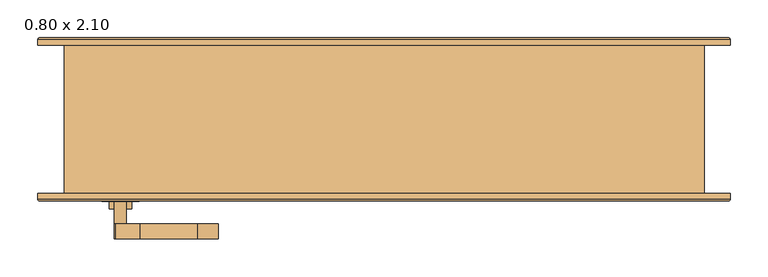
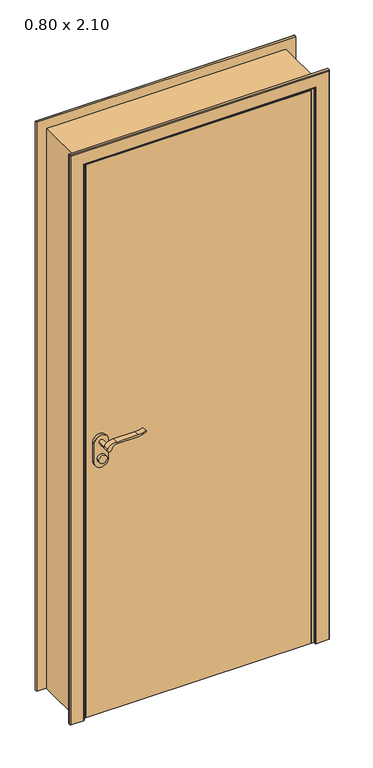
"""IFC4 building model written with IfcOpenShell, lengths in millimetres: door geometry, .CC_ND 300_PORTA SIMPLES DE ABRIR_COM EXTENSÃO : 0.80 x 2.10."""

import ifcopenshell
import ifcopenshell.guid

model = None  # the IFC model being written
_history = None  # IfcOwnerHistory: only IFC2X3 demands one
_inside = {}  # id of a spatial element -> (the spatial element, [elements in it])
_under = {}  # id of a project, library or spatial element -> (it, [spatial elements below it])
_declared = {}  # id of a project -> (the project, [libraries it declares])
_typed = {}  # id of a type object -> (the type object, [elements of that type])
_made_of = {}  # id of a material, layer set ... -> (it, [elements and type objects made of it])


def new_model(schema):
    """Start an empty IFC model of exactly this schema.

    Asked for "IFC4X3", IfcOpenShell would pick the latest addendum, in which some entities
    have other attributes; the version numbers below select the first issue.
    IFC2X3 requires an IfcOwnerHistory on every rooted entity: one is made here for all.
    """
    global model, _history
    if schema == "IFC4X3":
        model = ifcopenshell.file(schema_version=(4, 3, 0, 0))
    else:
        model = ifcopenshell.file(schema=schema)
    _inside.clear()
    _under.clear()
    _declared.clear()
    _typed.clear()
    _made_of.clear()
    _history = None
    if model.schema == "IFC2X3":
        org = make("IfcOrganization", Name="unknown")
        user = make(
            "IfcPersonAndOrganization",
            ThePerson=make("IfcPerson", FamilyName="unknown"),
            TheOrganization=org,
        )
        app = make(
            "IfcApplication",
            ApplicationDeveloper=org,
            Version="unknown",
            ApplicationFullName="unknown",
            ApplicationIdentifier="unknown",
        )
        _history = make(
            "IfcOwnerHistory",
            OwningUser=user,
            OwningApplication=app,
            ChangeAction="ADDED",
            CreationDate=0,
        )
    return model


def make(cls, **values):
    """One entity of the class cls with the attributes given. An attribute that is None is left unset."""
    return model.create_entity(
        cls, **{name: value for name, value in values.items() if value is not None}
    )


def rooted(cls, **values):
    """An entity with a GlobalId (a new one), such as an element, a storey or a relation."""
    return make(cls, GlobalId=ifcopenshell.guid.new(), OwnerHistory=_history, **values)


def si_unit(unit_type, name, prefix=None):
    """IfcSIUnit, for example si_unit("LENGTHUNIT", "METRE", prefix="MILLI")."""
    return make("IfcSIUnit", UnitType=unit_type, Prefix=prefix, Name=name)


def assignment(units):
    """IfcUnitAssignment: the units of a project."""
    return None if units is None else make("IfcUnitAssignment", Units=units)


def point(xyz):
    """IfcCartesianPoint."""
    return None if xyz is None else make("IfcCartesianPoint", Coordinates=xyz)


def direction(xyz):
    """IfcDirection."""
    return None if xyz is None else make("IfcDirection", DirectionRatios=xyz)


def frame(location, z_axis=None, x_axis=None):
    """IfcAxis2Placement3D, a coordinate frame: its origin and axes. An axis left out is left unset."""
    return make(
        "IfcAxis2Placement3D",
        Location=point(location),
        Axis=direction(z_axis),
        RefDirection=direction(x_axis),
    )


def frame_2d(location, x_axis=None):
    """IfcAxis2Placement2D, a coordinate frame in the plane: its origin and x axis."""
    return make(
        "IfcAxis2Placement2D", Location=point(location), RefDirection=direction(x_axis)
    )


def origin():
    """The frame at (0, 0, 0) with its axes left unset."""
    return frame((0.0, 0.0, 0.0))


def origin_with_axes():
    """The frame at (0, 0, 0) with the z axis (0, 0, 1) and the x axis (1, 0, 0) written out."""
    return frame((0.0, 0.0, 0.0), z_axis=(0.0, 0.0, 1.0), x_axis=(1.0, 0.0, 0.0))


def place(relative_to, where):
    """IfcLocalPlacement: puts the frame where relative to a parent placement (None: the world)."""
    return make(
        "IfcLocalPlacement", PlacementRelTo=relative_to, RelativePlacement=where
    )


def context(
    kind, dimensions, precision=None, world=None, true_north=None, identifier=None
):
    """IfcGeometricRepresentationContext, for example the 3D "Model" context."""
    return make(
        "IfcGeometricRepresentationContext",
        ContextIdentifier=identifier,
        ContextType=kind,
        CoordinateSpaceDimension=dimensions,
        Precision=precision,
        WorldCoordinateSystem=world,
        TrueNorth=true_north,
    )


def project(units=None, contexts=None):
    """IfcProject with its units and contexts."""
    return rooted(
        "IfcProject",
        Name="project",
        RepresentationContexts=contexts,
        UnitsInContext=assignment(units),
    )


def spatial(cls, under=None, at=None, **own):
    """A site, building, storey or space (cls), placed at a placement, below another one or the project."""
    s = rooted(cls, ObjectPlacement=at, **own)
    if under is not None:
        _under.setdefault(under.id(), (under, []))[1].append(s)
    return s


def polyline(points):
    """IfcPolyline through the points."""
    return make("IfcPolyline", Points=[point(p) for p in points])


def circle_curve(where, radius):
    """IfcCircle in the frame where."""
    return make("IfcCircle", Position=where, Radius=radius)


def ellipse_curve(where, semi_axis1, semi_axis2):
    """IfcEllipse in the frame where."""
    return make(
        "IfcEllipse", Position=where, SemiAxis1=semi_axis1, SemiAxis2=semi_axis2
    )


def trimmed(basis, trim1, trim2, sense, master):
    """IfcTrimmedCurve: the piece of a basis curve between two trims."""
    return make(
        "IfcTrimmedCurve",
        BasisCurve=basis,
        Trim1=trim1,
        Trim2=trim2,
        SenseAgreement=sense,
        MasterRepresentation=master,
    )


def segment(curve, same_sense, transition):
    """IfcCompositeCurveSegment."""
    return make(
        "IfcCompositeCurveSegment",
        Transition=transition,
        SameSense=same_sense,
        ParentCurve=curve,
    )


def composite_curve(segments, self_intersect=None):
    """IfcCompositeCurve: segments joined end to end."""
    return make("IfcCompositeCurve", Segments=segments, SelfIntersect=self_intersect)


def outline(outer, holes=None, kind="AREA"):
    """IfcArbitraryClosedProfileDef: a profile drawn as a closed curve; with holes, ...WithVoids."""
    if holes is None:
        return make("IfcArbitraryClosedProfileDef", ProfileType=kind, OuterCurve=outer)
    return make(
        "IfcArbitraryProfileDefWithVoids",
        ProfileType=kind,
        OuterCurve=outer,
        InnerCurves=holes,
    )


def extrude(swept, where, along, depth):
    """IfcExtrudedAreaSolid: the profile swept, set in the frame where, extruded along a direction by depth."""
    return make(
        "IfcExtrudedAreaSolid",
        SweptArea=swept,
        Position=where,
        ExtrudedDirection=direction(along),
        Depth=depth,
    )


def faces_of(points, faces, orient=None, outer=None):
    """IfcFace entities. A face is a list of loops; a loop is a list of indices into points, from 0.

    orient and outer hold one flag for each loop. By default every Orientation is true, the
    first loop of a face is its IfcFaceOuterBound and the others are IfcFaceBound.
    """
    made = []
    for i, loops in enumerate(faces):
        bounds = []
        for j, loop in enumerate(loops):
            is_outer = j == 0 if outer is None else outer[i][j]
            bounds.append(
                make(
                    "IfcFaceOuterBound" if is_outer else "IfcFaceBound",
                    Bound=make("IfcPolyLoop", Polygon=[points[k] for k in loop]),
                    Orientation=True if orient is None else orient[i][j],
                )
            )
        made.append(make("IfcFace", Bounds=bounds))
    return made


def faceted_brep(points, faces, orient=None, outer=None, voids=None):
    """IfcFacetedBrep: a solid bounded by flat faces; with voids (closed shells), ...WithVoids."""
    shared = [point(p) for p in points]
    hull = make("IfcClosedShell", CfsFaces=faces_of(shared, faces, orient, outer))
    if voids is None:
        return make("IfcFacetedBrep", Outer=hull)
    return make(
        "IfcFacetedBrepWithVoids",
        Outer=hull,
        Voids=[
            make(cls, CfsFaces=faces_of(shared, fs, o, b)) for cls, fs, o, b in voids
        ],
    )


def shape(context_of_items, identifier, shape_type, items):
    """IfcShapeRepresentation: the items that make up one representation, for example the "Body"."""
    return make(
        "IfcShapeRepresentation",
        ContextOfItems=context_of_items,
        RepresentationIdentifier=identifier,
        RepresentationType=shape_type,
        Items=items,
    )


def source(mapping_origin, context_of_items, identifier, shape_type, items):
    """IfcRepresentationMap: a shape defined once, which mapped items show again and again."""
    return make(
        "IfcRepresentationMap",
        MappingOrigin=mapping_origin,
        MappedRepresentation=shape(context_of_items, identifier, shape_type, items),
    )


def transform(
    local_origin,
    x_axis=None,
    y_axis=None,
    z_axis=None,
    scale=None,
    scale2=None,
    scale3=None,
    uniform=True,
):
    """IfcCartesianTransformationOperator3D, or its non-uniform kind. x_axis, y_axis, z_axis: its Axis1, 2, 3."""
    if uniform:
        return make(
            "IfcCartesianTransformationOperator3D",
            Axis1=direction(x_axis),
            Axis2=direction(y_axis),
            LocalOrigin=point(local_origin),
            Scale=scale,
            Axis3=direction(z_axis),
        )
    return make(
        "IfcCartesianTransformationOperator3DnonUniform",
        Axis1=direction(x_axis),
        Axis2=direction(y_axis),
        LocalOrigin=point(local_origin),
        Scale=scale,
        Axis3=direction(z_axis),
        Scale2=scale2,
        Scale3=scale3,
    )


def mapped(mapping_source, mapping_target):
    """IfcMappedItem: shows the shape of a source again, moved by a transform."""
    return make(
        "IfcMappedItem", MappingSource=mapping_source, MappingTarget=mapping_target
    )


def made_of(thing, what):
    """Note that an element or type object is made of a material, layer set ...; save() writes the relation."""
    if what is not None:
        _made_of.setdefault(what.id(), (what, []))[1].append(thing)
    return thing


def element(
    cls,
    number,
    at=None,
    inside=None,
    cuts=None,
    type_object=None,
    material=None,
    context=None,
    identifier="Body",
    shape_type=None,
    held_by="IfcProductDefinitionShape",
    body=None,
    shapes=None,
    **own,
):
    """One element of the class cls, such as IfcWall. Its Tag is "e" and its number.

    at: its placement. inside: the storey or other place that contains it. cuts: it is an
    opening in that element (IfcRelVoidsElement). A single representation is given by context,
    identifier, shape_type and body (its items); several are given by shapes. held_by: the class
    of the entity that holds the representations. save() writes the other relations.
    """
    e = rooted(cls, Tag="e%d" % number, ObjectPlacement=at, **own)
    if body is not None:
        shapes = [shape(context, identifier, shape_type, body)]
    if shapes is not None:
        e.Representation = make(held_by, Representations=shapes)
    if inside is not None:
        _inside.setdefault(inside.id(), (inside, []))[1].append(e)
    if cuts is not None:
        rooted(
            "IfcRelVoidsElement", RelatingBuildingElement=cuts, RelatedOpeningElement=e
        )
    if type_object is not None:
        _typed.setdefault(type_object.id(), (type_object, []))[1].append(e)
    return made_of(e, material)


def aggregate(whole, parts):
    """IfcRelAggregates: a whole, such as a stair, and the parts it consists of."""
    return rooted("IfcRelAggregates", RelatingObject=whole, RelatedObjects=parts)


def save(model, path):
    """Write the relations noted so far, then the file.

    IfcRelAggregates (storeys below a building ...), IfcRelContainedInSpatialStructure (elements
    in a storey), IfcRelDefinesByType, IfcRelAssociatesMaterial and IfcRelDeclares: one each for
    every whole, place, type object, material and project.
    """
    for whole, parts in _under.values():
        aggregate(whole, parts)
    for where, things in _inside.values():
        rooted(
            "IfcRelContainedInSpatialStructure",
            RelatedElements=things,
            RelatingStructure=where,
        )
    for kind, things in _typed.values():
        rooted("IfcRelDefinesByType", RelatedObjects=things, RelatingType=kind)
    for what, things in _made_of.values():
        rooted("IfcRelAssociatesMaterial", RelatedObjects=things, RelatingMaterial=what)
    for by, libraries in _declared.values():
        rooted("IfcRelDeclares", RelatingContext=by, RelatedDefinitions=libraries)
    model.write(path)


def plane_surface(at):
    """IfcPlane: the flat surface through the origin of the frame at, square to its z axis."""
    return make("IfcPlane", Position=at)


def cylinder_surface(at, radius):
    """IfcCylindricalSurface: all points at the distance radius from the z axis of the frame at."""
    return make("IfcCylindricalSurface", Position=at, Radius=radius)


def advanced_brep(points, edges, surfaces, faces):
    """IfcAdvancedBrep: a solid bounded by faces that lie on surfaces and meet in shared edges.

    An edge is (start, end): straight between two places in points (the first is 0);
    or (start, end, curve); or (start, end, curve, False) where it runs against its curve.
    A face is (place in surfaces, loops), or (place, loops, False) where it looks against
    its surface's normal. A loop lists edges by number (the first is 1), with a minus sign
    where the edge is run from its end to its start. The first loop is the outer one.
    """
    corners = [point(p) for p in points]
    vertices = [make("IfcVertexPoint", VertexGeometry=c) for c in corners]
    made = []
    for start, end, *more in edges:
        made.append(
            make(
                "IfcEdgeCurve",
                EdgeStart=vertices[start],
                EdgeEnd=vertices[end],
                EdgeGeometry=more[0] if more else make("IfcPolyline", Points=[corners[start], corners[end]]),
                SameSense=more[1] if len(more) > 1 else True,
            )
        )
    hull = []
    for where, loops, *sense in faces:
        bounds = []
        for j, loop in enumerate(loops):
            ring = [make("IfcOrientedEdge", EdgeElement=made[abs(k) - 1], Orientation=k > 0) for k in loop]
            bounds.append(
                make(
                    "IfcFaceOuterBound" if j == 0 else "IfcFaceBound",
                    Bound=make("IfcEdgeLoop", EdgeList=ring),
                    Orientation=True,
                )
            )
        hull.append(make("IfcAdvancedFace", Bounds=bounds, FaceSurface=surfaces[where], SameSense=sense[0] if sense else True))
    return make("IfcAdvancedBrep", Outer=make("IfcClosedShell", CfsFaces=hull))


def door_0_80_x_2_10_6c9b3ed6(model_context):
    return source(origin(), model_context, "Body", "SolidModel", [
        extrude(outline(composite_curve([segment(trimmed(circle_curve(frame_2d((964.5, -350.0)), 15.0), [point((964.5, -335.0))], [point((964.5, -365.0))], False, "CARTESIAN"), True, "CONTINUOUS"), segment(trimmed(circle_curve(frame_2d((964.5, -350.0)), 15.0), [point((964.5, -365.0))], [point((964.5, -335.0))], False, "CARTESIAN"), True, "CONTINUOUS")], self_intersect=False)), frame((0.0, -118.8, 0.0), z_axis=(0.0, 1.0, 0.0), x_axis=(0.0, 0.0, 1.0)), (0.0, 0.0, 1.0), 10.0),
        extrude(outline(composite_curve([segment(trimmed(circle_curve(frame_2d((964.5, -350.0)), 15.0), [point((964.5, -335.0))], [point((964.5, -365.0))], False, "CARTESIAN"), True, "CONTINUOUS"), segment(trimmed(circle_curve(frame_2d((964.5, -350.0)), 15.0), [point((964.5, -365.0))], [point((964.5, -335.0))], False, "CARTESIAN"), True, "CONTINUOUS")], self_intersect=False)), frame((0.0, -58.8, 0.0), z_axis=(0.0, 1.0, 0.0), x_axis=(0.0, 0.0, 1.0)), (0.0, 0.0, 1.0), 10.0),
        extrude(outline(composite_curve([segment(trimmed(circle_curve(frame_2d((1024.5, -350.0)), 8.0), [point((1029.1523287, -356.5081363))], [point((1024.5, -342.0))], False, "CARTESIAN"), True, "CONTINUOUS"), segment(trimmed(circle_curve(frame_2d((1019.3738613, -324.6138099)), 18.1261387), [point((1024.5, -342.0))], [point((1037.5, -324.6138099))], True, "CARTESIAN"), True, "CONTINUOUS"), segment(polyline([(1037.5, -324.6138099), (1037.5, -248.3564091)]), True, "CONTINUOUS"), segment(trimmed(circle_curve(frame_2d((1096.7709207, -251.9396612)), 59.3791355), [point((1037.5, -248.3564091))], [point((1046.7135558, -220.0))], False, "CARTESIAN"), True, "CONTINUOUS"), segment(polyline([(1046.7135558, -220.0), (1049.5, -220.0)]), True, "CONTINUOUS"), segment(trimmed(circle_curve(frame_2d((1127.7850638, -248.4227909)), 83.2850902), [point((1049.5, -220.0))], [point((1044.5, -248.3564091))], True, "CARTESIAN"), True, "CONTINUOUS"), segment(polyline([(1044.5, -248.3564091), (1044.5, -324.6325667)]), True, "CONTINUOUS"), segment(trimmed(circle_curve(frame_2d((1007.2555521, -326.3324871)), 37.2832219), [point((1044.5, -324.6325667))], [point((1029.1523287, -356.5081363))], False, "CARTESIAN"), True, "CONTINUOUS")], self_intersect=False)), frame((0.0, -158.8, 0.0), z_axis=(0.0, 1.0, 0.0), x_axis=(0.0, 0.0, 1.0)), (0.0, 0.0, 1.0), 20.0),
        extrude(outline(composite_curve([segment(trimmed(circle_curve(frame_2d((1019.3738682, -324.6138122)), 18.1261318), [point((1024.4999903, -342.0))], [point((1037.5, -324.6138122))], True, "CARTESIAN"), True, "CONTINUOUS"), segment(polyline([(1037.5, -324.6138122), (1037.5, -248.3564091)]), True, "CONTINUOUS"), segment(trimmed(circle_curve(frame_2d((1096.7709207, -251.9396612)), 59.3791355), [point((1037.5, -248.3564091))], [point((1046.7135558, -220.0))], False, "CARTESIAN"), True, "CONTINUOUS"), segment(polyline([(1046.7135558, -220.0), (1049.5, -220.0)]), True, "CONTINUOUS"), segment(trimmed(circle_curve(frame_2d((1127.7850638, -248.4227909)), 83.2850902), [point((1049.5, -220.0))], [point((1044.5, -248.3564091))], True, "CARTESIAN"), True, "CONTINUOUS"), segment(polyline([(1044.5, -248.3564091), (1044.5, -324.6325667)]), True, "CONTINUOUS"), segment(trimmed(circle_curve(frame_2d((1007.2555521, -326.3324871)), 37.2832219), [point((1044.5, -324.6325667))], [point((1029.1523287, -356.5081363))], False, "CARTESIAN"), True, "CONTINUOUS"), segment(trimmed(circle_curve(frame_2d((1024.5, -350.0)), 8.0), [point((1029.1523287, -356.5081363))], [point((1024.4999903, -342.0))], False, "CARTESIAN"), True, "CONTINUOUS")], self_intersect=False)), frame((0.0, -28.8, 0.0), z_axis=(0.0, 1.0, 0.0), x_axis=(0.0, 0.0, 1.0)), (0.0, 0.0, 1.0), 20.0),
        extrude(outline(composite_curve([segment(trimmed(circle_curve(frame_2d((1024.5, -350.0)), 8.0), [point((1024.5, -342.0))], [point((1024.5, -358.0))], False, "CARTESIAN"), True, "CONTINUOUS"), segment(trimmed(circle_curve(frame_2d((1024.5, -350.0)), 8.0), [point((1024.5, -358.0))], [point((1024.5, -342.0))], False, "CARTESIAN"), True, "CONTINUOUS")], self_intersect=False)), frame((0.0, -138.8, 0.0), z_axis=(0.0, 1.0, 0.0), x_axis=(0.0, 0.0, 1.0)), (0.0, 0.0, 1.0), 30.0),
        extrude(outline(composite_curve([segment(trimmed(circle_curve(frame_2d((1024.5, -350.0)), 8.0), [point((1024.5, -342.0))], [point((1024.5, -358.0))], False, "CARTESIAN"), True, "CONTINUOUS"), segment(trimmed(circle_curve(frame_2d((1024.5, -350.0)), 8.0), [point((1024.5, -358.0))], [point((1024.5, -342.0))], False, "CARTESIAN"), True, "CONTINUOUS")], self_intersect=False)), frame((0.0, -58.8, 0.0), z_axis=(0.0, 1.0, 0.0), x_axis=(0.0, 0.0, 1.0)), (0.0, 0.0, 1.0), 30.0),
        extrude(outline(composite_curve([segment(trimmed(circle_curve(frame_2d((954.5, -350.0)), 25.0), [point((954.5, -375.0))], [point((954.5, -325.0))], False, "CARTESIAN"), True, "CONTINUOUS"), segment(polyline([(954.5, -325.0), (1024.5, -325.0)]), True, "CONTINUOUS"), segment(trimmed(circle_curve(frame_2d((1024.5, -350.0)), 25.0), [point((1024.5, -325.0))], [point((1024.5, -375.0))], False, "CARTESIAN"), True, "CONTINUOUS"), segment(polyline([(1024.5, -375.0), (954.5, -375.0)]), True, "CONTINUOUS")], self_intersect=False)), frame((0.0, -108.8, 0.0), z_axis=(0.0, 1.0, 0.0), x_axis=(0.0, 0.0, 1.0)), (0.0, 0.0, 1.0), 10.0),
        extrude(outline(composite_curve([segment(trimmed(circle_curve(frame_2d((954.5, -350.0)), 25.0), [point((954.5, -375.0))], [point((954.5, -325.0))], False, "CARTESIAN"), True, "CONTINUOUS"), segment(polyline([(954.5, -325.0), (1024.5, -325.0)]), True, "CONTINUOUS"), segment(trimmed(circle_curve(frame_2d((1024.5, -350.0)), 25.0), [point((1024.5, -325.0))], [point((1024.5, -375.0))], False, "CARTESIAN"), True, "CONTINUOUS"), segment(polyline([(1024.5, -375.0), (954.5, -375.0)]), True, "CONTINUOUS")], self_intersect=False)), frame((0.0, -68.8, 0.0), z_axis=(0.0, 1.0, 0.0), x_axis=(0.0, 0.0, 1.0)), (0.0, 0.0, 1.0), 10.0),
        advanced_brep(
        [(-460.0, -98.8, 0.0), (-410.0, -98.8, 0.0), (-410.0, -105.8, 0.0), (-413.0, -108.8, 0.0), (-457.0, -108.8, 0.0), (-460.0, -105.8, 0.0), (-460.0, -98.8, 2135.0), (460.0, -98.8, 2135.0), (460.0, -98.8, 0.0), (410.0, -98.8, 0.0), (410.0, -98.8, 2085.0), (-410.0, -98.8, 2085.0), (-410.0, -105.8, 2085.0), (-413.0, -108.8, 2088.0), (413.0, -108.8, 2088.0), (413.0, -108.8, 0.0), (457.0, -108.8, 0.0), (457.0, -108.8, 2132.0), (-457.0, -108.8, 2132.0), (-460.0, -105.8, 2135.0), (460.0, -105.8, 2135.0), (460.0, -105.8, 0.0), (410.0, -105.8, 0.0), (410.0, -105.8, 2085.0)],
        [
            (0, 1),
            (1, 2),
            (2, 3, circle_curve(frame((-413.0, -105.8, 0.0), z_axis=(0.0, 0.0, -1.0), x_axis=(1.0, 0.0, 0.0)), 3.0)),
            (3, 4),
            (4, 5, circle_curve(frame((-457.0, -105.8, 0.0), z_axis=(0.0, 0.0, -1.0), x_axis=(1.0, 0.0, 0.0)), 3.0)),
            (5, 0),
            (0, 6),
            (6, 7),
            (7, 8),
            (8, 9),
            (9, 10),
            (10, 11),
            (11, 1),
            (11, 12),
            (12, 2),
            (12, 13, ellipse_curve(frame((-413.0, -105.8, 2088.0), z_axis=(-0.7071067811865475, 0.0, -0.7071067811865475), x_axis=(0.7071067811865474, 0.0, -0.7071067811865476)), 4.2426407, 3.0)),
            (13, 3),
            (13, 14),
            (14, 15),
            (15, 16),
            (16, 17),
            (17, 18),
            (18, 4),
            (18, 19, ellipse_curve(frame((-457.0, -105.8, 2132.0), z_axis=(-0.7071067811865475, 0.0, -0.7071067811865475), x_axis=(0.7071067811865474, 0.0, -0.7071067811865476)), 4.2426407, 3.0)),
            (19, 5),
            (19, 6),
            (7, 20),
            (20, 21),
            (21, 8),
            (21, 16, circle_curve(frame((457.0, -105.8, 0.0), z_axis=(0.0, 0.0, -1.0), x_axis=(-1.0, 0.0, 0.0)), 3.0)),
            (15, 22, circle_curve(frame((413.0, -105.8, 0.0), z_axis=(0.0, 0.0, -1.0), x_axis=(-1.0, 0.0, 0.0)), 3.0)),
            (22, 9),
            (23, 10),
            (22, 23),
            (14, 23, ellipse_curve(frame((413.0, -105.8, 2088.0), z_axis=(0.7071067811865475, 0.0, -0.7071067811865475), x_axis=(0.7071067811865474, 0.0, 0.7071067811865476)), 4.2426407, 3.0)),
            (20, 17, ellipse_curve(frame((457.0, -105.8, 2132.0), z_axis=(0.7071067811865475, 0.0, -0.7071067811865475), x_axis=(0.7071067811865474, 0.0, 0.7071067811865476)), 4.2426407, 3.0)),
            (23, 12),
            (19, 20),
        ],
        [
            plane_surface(frame((-410.0, -98.8, 0.0), z_axis=(0.0, 0.0, -1.0), x_axis=(0.0, 1.0, 0.0))),
            plane_surface(frame((-460.0, -98.8, 0.0), z_axis=(0.0, 1.0, 0.0), x_axis=(0.0, 0.0, 1.0))),
            plane_surface(frame((-410.0, -98.8, 0.0), z_axis=(1.0, 0.0, 0.0), x_axis=(0.0, 0.0, 1.0))),
            cylinder_surface(frame((-413.0, -105.8, 0.0), z_axis=(0.0, 0.0, -1.0), x_axis=(1.0, 0.0, 0.0)), 3.0),
            plane_surface(frame((-413.0, -108.8, 0.0), z_axis=(0.0, -1.0, 0.0), x_axis=(0.0, 0.0, 1.0))),
            cylinder_surface(frame((-457.0, -105.8, 0.0), z_axis=(0.0, 0.0, -1.0), x_axis=(1.0, 0.0, 0.0)), 3.0),
            plane_surface(frame((-460.0, -105.8, 0.0), z_axis=(-1.0, 0.0, 0.0), x_axis=(0.0, 0.0, 1.0))),
            plane_surface(frame((460.0, -105.8, 2135.0), z_axis=(1.0, 0.0, 0.0), x_axis=(0.0, 0.0, -1.0))),
            plane_surface(frame((410.0, -98.8, 0.0), z_axis=(0.0, 0.0, -1.0), x_axis=(0.0, 1.0, 0.0))),
            plane_surface(frame((410.0, -98.8, 2085.0), z_axis=(-1.0, 0.0, 0.0), x_axis=(0.0, 0.0, -1.0))),
            cylinder_surface(frame((413.0, -105.8, 2085.0), z_axis=(0.0, 0.0, 1.0), x_axis=(-1.0, 0.0, 0.0)), 3.0),
            cylinder_surface(frame((457.0, -105.8, 2085.0), z_axis=(0.0, 0.0, 1.0), x_axis=(-1.0, 0.0, 0.0)), 3.0),
            plane_surface(frame((-410.0, -98.8, 2085.0), z_axis=(0.0, 0.0, -1.0), x_axis=(1.0, 0.0, 0.0))),
            plane_surface(frame((-460.0, -105.8, 2135.0), z_axis=(0.0, 0.0, 1.0), x_axis=(1.0, 0.0, 0.0))),
            cylinder_surface(frame((-410.0, -105.8, 2088.0), z_axis=(-1.0, 0.0, 0.0), x_axis=(0.0, 0.0, -1.0)), 3.0),
            cylinder_surface(frame((-410.0, -105.8, 2132.0), z_axis=(-1.0, 0.0, 0.0), x_axis=(0.0, 0.0, -1.0)), 3.0),
        ],
        [
            (0, [[1, 2, 3, 4, 5, 6]]),
            (1, [[-1, 7, 8, 9, 10, 11, 12, 13]]),
            (2, [[-2, -13, 14, 15]]),
            (3, [[-3, -15, 16, 17]]),
            (4, [[-4, -17, 18, 19, 20, 21, 22, 23]]),
            (5, [[-5, -23, 24, 25]]),
            (6, [[-6, -25, 26, -7]]),
            (7, [[27, 28, 29, -9]]),
            (8, [[-29, 30, -20, 31, 32, -10]]),
            (9, [[33, -11, -32, 34]]),
            (10, [[35, -34, -31, -19]]),
            (11, [[36, -21, -30, -28]]),
            (12, [[-14, -12, -33, 37]]),
            (13, [[-26, 38, -27, -8]]),
            (14, [[-16, -37, -35, -18]]),
            (15, [[-24, -22, -36, -38]]),
        ],
    ),
        advanced_brep(
        [(460.0, 98.8, 0.0), (410.0, 98.8, 0.0), (410.0, 105.8157283, 0.0), (412.9842717, 108.8, 0.0), (457.0342217, 108.8, 0.0), (460.0, 105.8342217, 0.0), (460.0, 98.8, 2135.0), (-460.0, 98.8, 2135.0), (-460.0, 98.8, 0.0), (-410.0, 98.8, 0.0), (-410.0, 98.8, 2085.0), (410.0, 98.8, 2085.0), (410.0, 105.8157283, 2085.0), (412.9842717, 108.8, 2087.9842717), (-412.9842717, 108.8, 2087.9842717), (-412.9842717, 108.8, 0.0), (-457.0342217, 108.8, 0.0), (-457.0342217, 108.8, 2132.0342217), (457.0342217, 108.8, 2132.0342217), (460.0, 105.8342217, 2135.0), (-460.0, 105.8342217, 2135.0), (-460.0, 105.8342217, 0.0), (-410.0, 105.8157283, 0.0), (-410.0, 105.8157283, 2085.0)],
        [
            (0, 1),
            (1, 2),
            (2, 3, circle_curve(frame((412.9842717, 105.8157283, 0.0), z_axis=(0.0, 0.0, -1.0), x_axis=(1.0, 0.0, 0.0)), 2.9842717)),
            (3, 4),
            (4, 5, circle_curve(frame((457.0342217, 105.8342217, 0.0), z_axis=(0.0, 0.0, -1.0), x_axis=(1.0, 0.0, 0.0)), 2.9657783)),
            (5, 0),
            (0, 6),
            (6, 7),
            (7, 8),
            (8, 9),
            (9, 10),
            (10, 11),
            (11, 1),
            (11, 12),
            (12, 2),
            (12, 13, ellipse_curve(frame((412.9842717, 105.8157283, 2087.9842717), z_axis=(0.7071067811865475, 0.0, -0.7071067811865475), x_axis=(-0.7071067811865474, 0.0, -0.7071067811865476)), 4.2203975, 2.9842717)),
            (13, 3),
            (13, 14),
            (14, 15),
            (15, 16),
            (16, 17),
            (17, 18),
            (18, 4),
            (18, 19, ellipse_curve(frame((457.0342217, 105.8342217, 2132.0342217), z_axis=(0.7071067811865475, 0.0, -0.7071067811865475), x_axis=(-0.7071067811865474, 0.0, -0.7071067811865476)), 4.1942438, 2.9657783)),
            (19, 5),
            (19, 6),
            (7, 20),
            (20, 21),
            (21, 8),
            (21, 16, circle_curve(frame((-457.0342217, 105.8342217, 0.0), z_axis=(0.0, 0.0, -1.0), x_axis=(-1.0, 0.0, 0.0)), 2.9657783)),
            (15, 22, circle_curve(frame((-412.9842717, 105.8157283, 0.0), z_axis=(0.0, 0.0, -1.0), x_axis=(-1.0, 0.0, 0.0)), 2.9842717)),
            (22, 9),
            (23, 10),
            (22, 23),
            (14, 23, ellipse_curve(frame((-412.9842717, 105.8157283, 2087.9842717), z_axis=(-0.7071067811865475, 0.0, -0.7071067811865475), x_axis=(-0.7071067811865474, 0.0, 0.7071067811865476)), 4.2203975, 2.9842717)),
            (20, 17, ellipse_curve(frame((-457.0342217, 105.8342217, 2132.0342217), z_axis=(-0.7071067811865475, 0.0, -0.7071067811865475), x_axis=(-0.7071067811865474, 0.0, 0.7071067811865476)), 4.1942438, 2.9657783)),
            (23, 12),
            (19, 20),
        ],
        [
            plane_surface(frame((410.0, 98.8, 0.0), z_axis=(0.0, 0.0, -1.0), x_axis=(0.0, 1.0, 0.0))),
            plane_surface(frame((460.0, 98.8, 0.0), z_axis=(0.0, -1.0, 0.0), x_axis=(0.0, 0.0, 1.0))),
            plane_surface(frame((410.0, 98.8, 0.0), z_axis=(-1.0, 0.0, 0.0), x_axis=(0.0, 0.0, 1.0))),
            cylinder_surface(frame((412.9842717, 105.8157283, 0.0), z_axis=(0.0, 0.0, -1.0), x_axis=(1.0, 0.0, 0.0)), 2.9842717),
            plane_surface(frame((412.9842717, 108.8, 0.0), z_axis=(0.0, 1.0, 0.0), x_axis=(0.0, 0.0, 1.0))),
            cylinder_surface(frame((457.0342217, 105.8342217, 0.0), z_axis=(0.0, 0.0, -1.0), x_axis=(1.0, 0.0, 0.0)), 2.9657783),
            plane_surface(frame((460.0, 105.8342217, 0.0), z_axis=(1.0, 0.0, 0.0), x_axis=(0.0, 0.0, 1.0))),
            plane_surface(frame((-460.0, 105.8342217, 2135.0), z_axis=(-1.0, 0.0, 0.0), x_axis=(0.0, 0.0, -1.0))),
            plane_surface(frame((-410.0, 98.8, 0.0), z_axis=(0.0, 0.0, -1.0), x_axis=(0.0, 1.0, 0.0))),
            plane_surface(frame((-410.0, 98.8, 2085.0), z_axis=(1.0, 0.0, 0.0), x_axis=(0.0, 0.0, -1.0))),
            cylinder_surface(frame((-412.9842717, 105.8157283, 2085.0), z_axis=(0.0, 0.0, 1.0), x_axis=(-1.0, 0.0, 0.0)), 2.9842717),
            cylinder_surface(frame((-457.0342217, 105.8342217, 2085.0), z_axis=(0.0, 0.0, 1.0), x_axis=(-1.0, 0.0, 0.0)), 2.9657783),
            plane_surface(frame((410.0, 98.8, 2085.0), z_axis=(0.0, 0.0, -1.0), x_axis=(-1.0, 0.0, 0.0))),
            plane_surface(frame((460.0, 105.8342217, 2135.0), z_axis=(0.0, 0.0, 1.0), x_axis=(-1.0, 0.0, 0.0))),
            cylinder_surface(frame((410.0, 105.8157283, 2087.9842717), z_axis=(1.0, 0.0, 0.0), x_axis=(0.0, 0.0, 1.0)), 2.9842717),
            cylinder_surface(frame((410.0, 105.8342217, 2132.0342217), z_axis=(1.0, 0.0, 0.0), x_axis=(0.0, 0.0, 1.0)), 2.9657783),
        ],
        [
            (0, [[1, 2, 3, 4, 5, 6]]),
            (1, [[-1, 7, 8, 9, 10, 11, 12, 13]]),
            (2, [[-2, -13, 14, 15]]),
            (3, [[-3, -15, 16, 17]]),
            (4, [[-4, -17, 18, 19, 20, 21, 22, 23]]),
            (5, [[-5, -23, 24, 25]]),
            (6, [[-6, -25, 26, -7]]),
            (7, [[27, 28, 29, -9]]),
            (8, [[-29, 30, -20, 31, 32, -10]]),
            (9, [[33, -11, -32, 34]]),
            (10, [[35, -34, -31, -19]]),
            (11, [[36, -21, -30, -28]]),
            (12, [[-14, -12, -33, 37]]),
            (13, [[-26, 38, -27, -8]]),
            (14, [[-16, -37, -35, -18]]),
            (15, [[-24, -22, -36, -38]]),
        ],
    ),
        faceted_brep([(392.0, 98.8, 0.0), (425.0, 98.8, 0.0), (425.0, -98.8, 0.0), (400.0, -98.8, 0.0), (400.0, -68.8, 0.0), (392.0, -68.8, 0.0), (392.0, 98.8, 2067.0), (-392.0, 98.8, 2067.0), (-392.0, 98.8, 0.0), (-425.0, 98.8, 0.0), (-425.0, 98.8, 2100.0), (425.0, 98.8, 2100.0), (425.0, -98.8, 2100.0), (-425.0, -98.8, 2100.0), (-425.0, -98.8, 0.0), (-400.0, -98.8, 0.0), (-400.0, -98.8, 2075.0), (400.0, -98.8, 2075.0), (400.0, -68.8, 2075.0), (-400.0, -68.8, 2075.0), (-400.0, -68.8, 0.0), (-392.0, -68.8, 0.0), (-392.0, -68.8, 2067.0), (392.0, -68.8, 2067.0)], [[[0, 1, 2, 3, 4, 5]], [[1, 0, 6, 7, 8, 9, 10, 11]], [[2, 1, 11, 12]], [[3, 2, 12, 13, 14, 15, 16, 17]], [[4, 3, 17, 18]], [[5, 4, 18, 19, 20, 21, 22, 23]], [[0, 5, 23, 6]], [[7, 22, 21, 8]], [[8, 21, 20, 15, 14, 9]], [[13, 10, 9, 14]], [[19, 16, 15, 20]], [[12, 11, 10, 13]], [[18, 17, 16, 19]], [[6, 23, 22, 7]]]),
        extrude(outline(polyline([(-400.0, -68.8), (400.0, -68.8), (400.0, -98.8), (-400.0, -98.8), (-400.0, -68.8)])), origin_with_axes(), (0.0, 0.0, 1.0), 2075.0),
    ])


if __name__ == "__main__":
    model = new_model("IFC4")
    model_context = context("Model", 3, world=origin())
    ifc_project = project(units=[si_unit("LENGTHUNIT", "METRE", prefix="MILLI")], contexts=[model_context])
    site = spatial("IfcSite", under=ifc_project)
    building = spatial("IfcBuilding", under=site)
    placement = place(None, origin())
    door_0_80_x_2_10_shape = door_0_80_x_2_10_6c9b3ed6(model_context)
    element("IfcDoor", 1, ObjectType=".CC_ND 300_PORTA SIMPLES DE ABRIR_COM EXTENSÃO : 0.80 x 2.10", at=placement, inside=building, context=model_context, shape_type="MappedRepresentation", body=[
        mapped(door_0_80_x_2_10_shape, transform((0.0, 0.0, 0.0), x_axis=(1.0, 0.0, 0.0), y_axis=(0.0, 1.0, 0.0), z_axis=(0.0, 0.0, 1.0))),
    ])
    save(model, "model.ifc")

# Revit data of these elements
# Type ".CC_ND 300_PORTA SIMPLES DE ABRIR_COM EXTENSÃO : 0.80 x 2.10"
#   Type Mark = "153"
#   Rough Width = 0.85 m
#   Espessura moldura externa = 0.01 m
#   Espessura moldura interna = 0.01 m
#   Largura moldura = 0.05 m
#   Extensão acabamento exterior [instance default] = 0.00 m
#   Extensão acabamento interior [instance default] = 0.00 m
#   Espessura batente = 0.025 m
#   Thickness = 0.03 m
#   Altura batente = 2.085 m
#   Aux Arco [instance default] = 0.80 m
#   Rough Height = 2.125 m
#   Height = 2.10 m
#   Width = 0.80 m
#   Moldura interna [instance default] = yes
#   Moldura externa [instance default] = yes
#   Porta = .MADEIRA COM PINTURA ESMALTE BRANCO ACETINADO
#   Moldura = .MADEIRA COM PINTURA ESMALTE BRANCO ACETINADO
#   Maçaneta = .ALUMÍNIO
#   Batente = .MADEIRA COM PINTURA ESMALTE BRANCO ACETINADO
#   Function = (empty or 0)
#   Wall Closure = (empty or 0)
# Element 1 (IfcDoor, ".CC_ND 300_PORTA SIMPLES DE ABRIR_COM EXTENSÃO : 0.80 x 2.10")
#   Materials on its faces: ".MADEIRA COM PINTURA ESMALTE BRANCO ACETINADO", ".ALUMÍNIO"
# Materials
#   ".MADEIRA COM PINTURA ESMALTE BRANCO ACETINADO": class ".CC_MADEIRAS", colour RGB 240 240 240, transparency 0, Description = "Madeira com pintura esmalte branco acetinado.", Cost = 0
#   ".ALUMÍNIO": class "CC_METAIS", colour RGB 244 244 244, transparency 0, Description = "Material alumínio", Cost = 0
